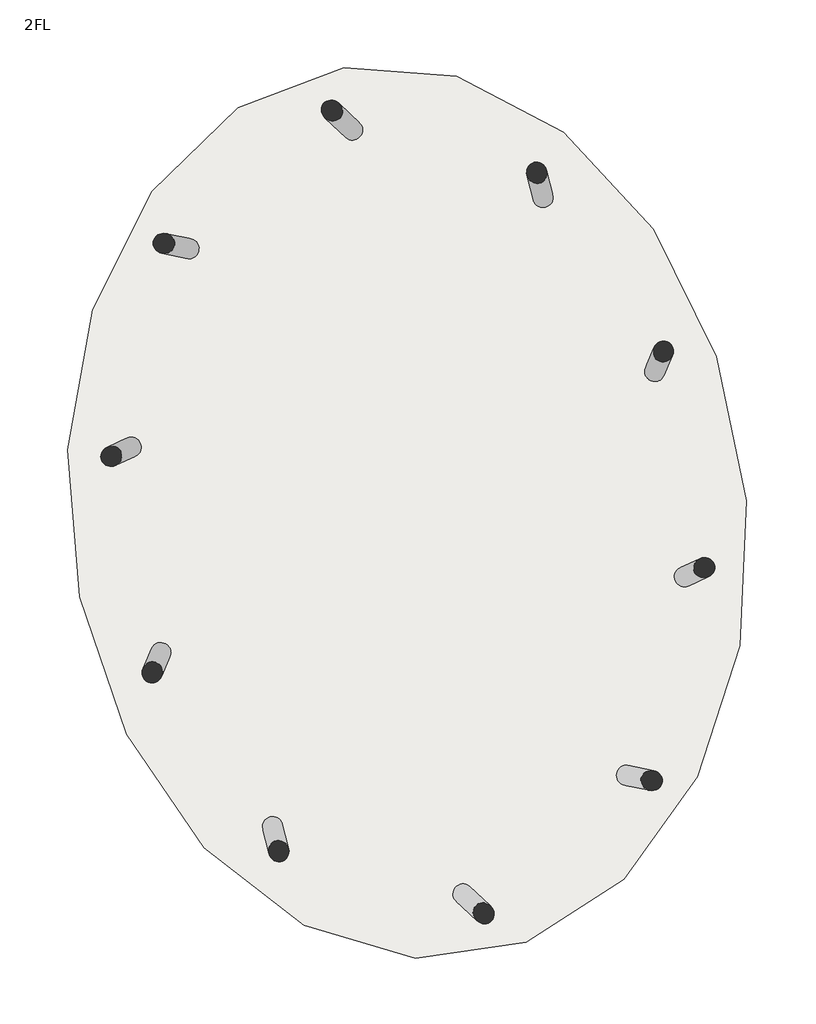
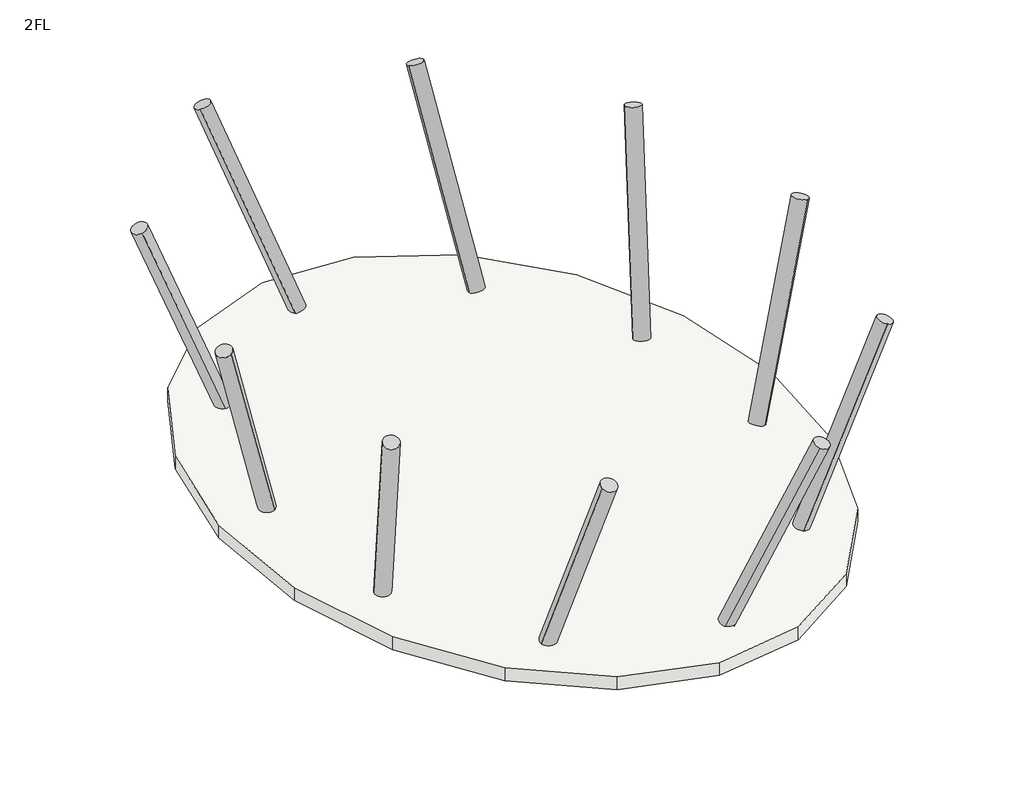
# One storey: 10 columns, 1 slab.
"""IFC4 building model written with IfcOpenShell, lengths in millimetres."""

from ifc_helpers import new_model, si_unit, point, frame, frame_2d, origin, place, context, project, spatial, polyline, circle_curve, trimmed, segment, composite_curve, outline, extrude, element, save

model = new_model("IFC4")

# Units and contexts
model_context = context("Model", 3, world=origin())
ifc_project = project(units=[si_unit("LENGTHUNIT", "METRE", prefix="MILLI")], contexts=[model_context])

# Site, building, storey
site = spatial("IfcSite", under=ifc_project)
building = spatial("IfcBuilding", under=site)
storey = spatial("IfcBuildingStorey", under=building, Name="2FL", Elevation=4500.0)

# Columns
placement = place(None, origin())
element("IfcColumn", 1, ObjectType="コンクリート-円形-柱 : 750", at=placement, inside=storey, context=model_context, shape_type="SweptSolid", body=[
    extrude(outline(composite_curve([segment(trimmed(circle_curve(frame_2d((0.0, -175.0)), 175.0), [point((0.0, -350.0))], [point((0.0, 0.0))], False, "CARTESIAN"), True, "CONTINUOUS"), segment(trimmed(circle_curve(frame_2d((0.0, -175.0)), 175.0), [point((0.0, 0.0))], [point((0.0, -350.0))], False, "CARTESIAN"), True, "CONTINUOUS")], self_intersect=False)), frame((-1071.9732491, 6494.7601075, 4500.0), z_axis=(-0.28099078546265055, 0.26401293669721404, 0.9226816069162731), x_axis=(-0.6724327329372604, 0.6318034246631801, -0.3855627734343714)), (0.0, 0.0, 1.0), 4877.088658),
])
element("IfcColumn", 2, ObjectType="コンクリート-円形-柱 : 750", at=placement, inside=storey, context=model_context, shape_type="SweptSolid", body=[
    extrude(outline(composite_curve([segment(trimmed(circle_curve(frame_2d((0.0, -175.0)), 175.0), [point((-1e-07, -350.0))], [point((0.0, 0.0))], False, "CARTESIAN"), True, "CONTINUOUS"), segment(trimmed(circle_curve(frame_2d((0.0, -175.0)), 175.0), [point((0.0, 0.0))], [point((-1e-07, -350.0))], False, "CARTESIAN"), True, "CONTINUOUS")], self_intersect=False)), frame((-3826.6258391, 4396.9020989, 4500.0), z_axis=(-0.34635425988715723, 0.07163495042837917, 0.9353647205957383), x_axis=(-0.9159785288994069, 0.18944786916305437, -0.3536846610539631)), (0.0, 0.0, 1.0), 4810.9575879),
])
element("IfcColumn", 3, ObjectType="コンクリート-円形-柱 : 750", at=placement, inside=storey, context=model_context, shape_type="SweptSolid", body=[
    extrude(outline(composite_curve([segment(trimmed(circle_curve(frame_2d((1e-07, -175.0)), 175.0), [point((1e-07, -350.0))], [point((0.0, 0.0))], False, "CARTESIAN"), True, "CONTINUOUS"), segment(trimmed(circle_curve(frame_2d((1e-07, -175.0)), 175.0), [point((0.0, 0.0))], [point((1e-07, -350.0))], False, "CARTESIAN"), True, "CONTINUOUS")], self_intersect=False)), frame((-4725.8996014, 968.4061468, 4500.0), z_axis=(-0.2766048317264904, -0.12727624729160697, 0.9525179914001235), x_axis=(-0.8653083333838384, -0.3981607867651079, -0.3044823082858417)), (0.0, 0.0, 1.0), 4724.320213),
])
element("IfcColumn", 4, ObjectType="コンクリート-円形-柱 : 750", at=placement, inside=storey, context=model_context, shape_type="SweptSolid", body=[
    extrude(outline(composite_curve([segment(trimmed(circle_curve(frame_2d((0.0, -174.9999999)), 175.0), [point((0.0, -350.0))], [point((0.0, 0.0))], False, "CARTESIAN"), True, "CONTINUOUS"), segment(trimmed(circle_curve(frame_2d((0.0, -174.9999999)), 175.0), [point((0.0, 0.0))], [point((0.0, -350.0))], False, "CARTESIAN"), True, "CONTINUOUS")], self_intersect=False)), frame((-4126.3500867, -2503.0860128, 4500.0), z_axis=(-0.11970297842291827, -0.2774723454322871, 0.9532472368053254), x_axis=(-0.37759676111988827, -0.8752719465793235, -0.3021915047168138)), (0.0, 0.0, 1.0), 4720.7060489),
])
element("IfcColumn", 5, ObjectType="コンクリート-円形-柱 : 750", at=placement, inside=storey, context=model_context, shape_type="SweptSolid", body=[
    extrude(outline(composite_curve([segment(trimmed(circle_curve(frame_2d((0.0, -175.0000001)), 175.0), [point((0.0, -350.0000001))], [point((0.0, 0.0))], False, "CARTESIAN"), True, "CONTINUOUS"), segment(trimmed(circle_curve(frame_2d((0.0, -175.0000001)), 175.0), [point((0.0, 0.0))], [point((0.0, -350.0000001))], False, "CARTESIAN"), True, "CONTINUOUS")], self_intersect=False)), frame((-2180.9908041, -5408.1479385, 4500.0), z_axis=(0.08649067637560048, -0.3396986048979982, 0.936549102145982), x_axis=(0.23108231127587697, -0.9075930729935325, -0.3505364164670415)), (0.0, 0.0, 1.0), 4804.8735412),
])
element("IfcColumn", 6, ObjectType="コンクリート-円形-柱 : 750", at=placement, inside=storey, context=model_context, shape_type="SweptSolid", body=[
    extrude(outline(composite_curve([segment(trimmed(circle_curve(frame_2d((1e-07, -175.0)), 175.0), [point((0.0, -349.9999999))], [point((0.0, 0.0))], False, "CARTESIAN"), True, "CONTINUOUS"), segment(trimmed(circle_curve(frame_2d((1e-07, -175.0)), 175.0), [point((0.0, 0.0))], [point((0.0, -349.9999999))], False, "CARTESIAN"), True, "CONTINUOUS")], self_intersect=False)), frame((1071.9732835, -6494.760113, 4500.0), z_axis=(0.28099078572078173, -0.2640129362256759, 0.9226816069725866), x_axis=(0.6724327338310597, -0.6318034237941437, -0.38556277329960825)), (0.0, 0.0, 1.0), 4877.088658),
])
element("IfcColumn", 7, ObjectType="コンクリート-円形-柱 : 750", at=placement, inside=storey, context=model_context, shape_type="SweptSolid", body=[
    extrude(outline(composite_curve([segment(trimmed(circle_curve(frame_2d((0.0, -175.0000001)), 175.0), [point((0.0, -350.0000001))], [point((0.0, 0.0))], False, "CARTESIAN"), True, "CONTINUOUS"), segment(trimmed(circle_curve(frame_2d((0.0, -175.0000001)), 175.0), [point((0.0, 0.0))], [point((0.0, -350.0000001))], False, "CARTESIAN"), True, "CONTINUOUS")], self_intersect=False)), frame((3826.6258503, -4396.9020689, 4500.0), z_axis=(0.3463542550375442, -0.07163494939228095, 0.9353647224708409), x_axis=(0.9159785307529951, -0.1894478694589561, -0.3536846560950119)), (0.0, 0.0, 1.0), 4810.9575783),
])
element("IfcColumn", 8, ObjectType="コンクリート-円形-柱 : 750", at=placement, inside=storey, context=model_context, shape_type="SweptSolid", body=[
    extrude(outline(composite_curve([segment(trimmed(circle_curve(frame_2d((0.0, -175.0)), 175.0), [point((0.0, -350.0))], [point((0.0, 0.0))], False, "CARTESIAN"), True, "CONTINUOUS"), segment(trimmed(circle_curve(frame_2d((0.0, -175.0)), 175.0), [point((0.0, 0.0))], [point((0.0, -350.0))], False, "CARTESIAN"), True, "CONTINUOUS")], self_intersect=False)), frame((4725.8995856, -968.4061159, 4500.0), z_axis=(0.2766048308454384, 0.12727624582018285, 0.9525179918525879), x_axis=(0.8653083350612423, 0.3981607842020958, -0.3044823068703882)), (0.0, 0.0, 1.0), 4724.320213),
])
element("IfcColumn", 9, ObjectType="コンクリート-円形-柱 : 750", at=placement, inside=storey, context=model_context, shape_type="SweptSolid", body=[
    extrude(outline(composite_curve([segment(trimmed(circle_curve(frame_2d((0.0, -175.0)), 175.0), [point((0.0, -350.0))], [point((0.0, 0.0))], False, "CARTESIAN"), True, "CONTINUOUS"), segment(trimmed(circle_curve(frame_2d((0.0, -175.0)), 175.0), [point((0.0, 0.0))], [point((0.0, -350.0))], False, "CARTESIAN"), True, "CONTINUOUS")], self_intersect=False)), frame((4126.3500785, 2503.0860416, 4500.0), z_axis=(0.11970297990658751, 0.2774723409819016, 0.9532472379144387), x_axis=(0.3775967706110317, 0.8752719436927168, -0.30219150121817384)), (0.0, 0.0, 1.0), 4720.7060489),
])
element("IfcColumn", 10, ObjectType="コンクリート-円形-柱 : 750", at=placement, inside=storey, context=model_context, shape_type="SweptSolid", body=[
    extrude(outline(composite_curve([segment(trimmed(circle_curve(frame_2d((0.0, -175.0)), 175.0), [point((0.0, -349.9999999))], [point((0.0, 0.0))], False, "CARTESIAN"), True, "CONTINUOUS"), segment(trimmed(circle_curve(frame_2d((0.0, -175.0)), 175.0), [point((0.0, 0.0))], [point((0.0, -349.9999999))], False, "CARTESIAN"), True, "CONTINUOUS")], self_intersect=False)), frame((2180.9907904, 5408.1479633, 4500.0), z_axis=(-0.08649067141484335, 0.33969860553455505, 0.9365491023732223), x_axis=(-0.23108229847823059, 0.907593076486432, -0.3505364158599098)), (0.0, 0.0, 1.0), 4804.8735412),
])

# Slab
element("IfcSlab", 11, ObjectType="一般 300 mm", at=placement, inside=storey, context=model_context, shape_type="SweptSolid", body=[
    extrude(outline(polyline([(-4452.1382845, 5562.8231985), (-2943.5413191, 7019.3874272), (-1109.0368535, 7713.5207453), (846.7172459, 7564.3443375), (2704.5669986, 6591.8020747), (4264.0133489, 4907.9851265), (5361.011627, 2697.322972), (5880.431389, 197.4886744), (5767.1640973, -2323.9978465), (5031.8877448, -4597.3352871), (3749.847008, -6377.7964465), (2055.0242208, -7469.0723164), (132.4995401, -7745.4896202), (-1801.1189579, -7175.9048715), (-3532.8419107, -5828.7575067), (-4878.8075864, -3854.6575012), (-5697.8715862, -1467.2199737), (-5903.7766886, 1077.6909267), (-5474.0300462, 3507.8658603), (-4452.1382845, 5562.8231985)])), frame((0.0, 0.0, 4200.0), z_axis=(0.0, 0.0, 1.0), x_axis=(1.0, 0.0, 0.0)), (0.0, 0.0, 1.0), 300.0),
])

save(model, "model.ifc")

# Revit data of these elements
# Type "コンクリート-円形-柱 : 750"
#   Keynote = "03310.Q1"
#   R = 350 mm
#   Structural Material [instance default] = コンクリート - 現場打ち
# Type "一般 300 mm"
#   Function = 0
#   Layers, outside or top first: 300 mm no material (function 1)
# Elements 1, 2, 3, 4, 5, 6, 7, 8, 9, 10 (IfcColumn, "コンクリート-円形-柱 : 750")
#   Structural Material = コンクリート - 現場打ち
#   Phase Created = 新しい建設
#   Materials on its faces: "コンクリート - 現場打ち"
# Element 11 (IfcSlab, "一般 300 mm")
#   Height Offset From Level = 0 mm
#   Phase Created = 新しい建設
# Materials
#   "コンクリート - 現場打ち": class "コンクリート", colour RGB 192 192 192, transparency 0
